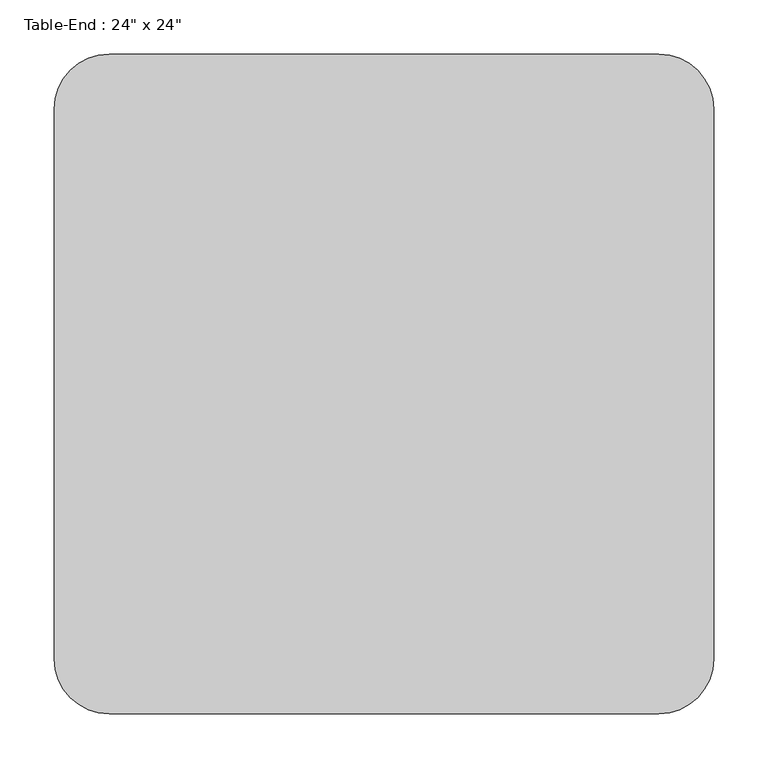
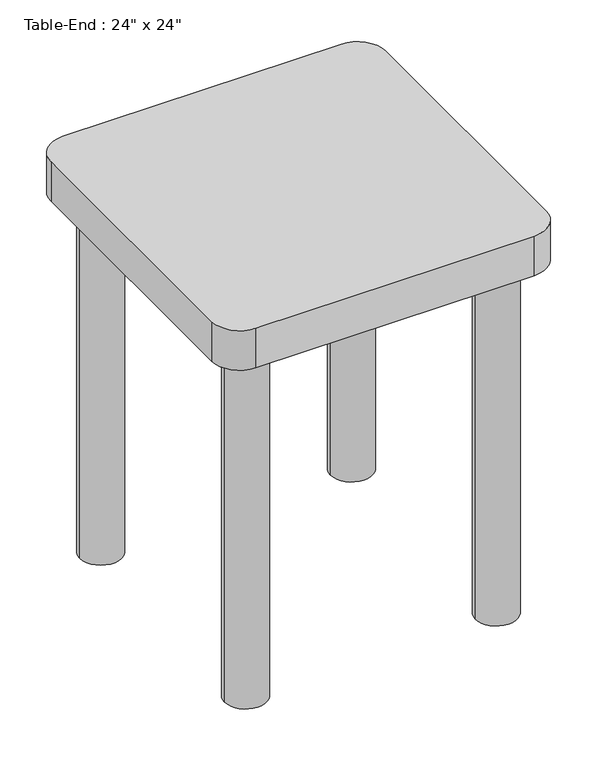
"""IFC4 building model written with IfcOpenShell, lengths in millimetres: furniture geometry."""

import ifcopenshell
import ifcopenshell.guid

model = None  # the IFC model being written
_history = None  # IfcOwnerHistory: only IFC2X3 demands one
_inside = {}  # id of a spatial element -> (the spatial element, [elements in it])
_under = {}  # id of a project, library or spatial element -> (it, [spatial elements below it])
_declared = {}  # id of a project -> (the project, [libraries it declares])
_typed = {}  # id of a type object -> (the type object, [elements of that type])
_made_of = {}  # id of a material, layer set ... -> (it, [elements and type objects made of it])


def new_model(schema):
    """Start an empty IFC model of exactly this schema.

    Asked for "IFC4X3", IfcOpenShell would pick the latest addendum, in which some entities
    have other attributes; the version numbers below select the first issue.
    IFC2X3 requires an IfcOwnerHistory on every rooted entity: one is made here for all.
    """
    global model, _history
    if schema == "IFC4X3":
        model = ifcopenshell.file(schema_version=(4, 3, 0, 0))
    else:
        model = ifcopenshell.file(schema=schema)
    _inside.clear()
    _under.clear()
    _declared.clear()
    _typed.clear()
    _made_of.clear()
    _history = None
    if model.schema == "IFC2X3":
        org = make("IfcOrganization", Name="unknown")
        user = make(
            "IfcPersonAndOrganization",
            ThePerson=make("IfcPerson", FamilyName="unknown"),
            TheOrganization=org,
        )
        app = make(
            "IfcApplication",
            ApplicationDeveloper=org,
            Version="unknown",
            ApplicationFullName="unknown",
            ApplicationIdentifier="unknown",
        )
        _history = make(
            "IfcOwnerHistory",
            OwningUser=user,
            OwningApplication=app,
            ChangeAction="ADDED",
            CreationDate=0,
        )
    return model


def make(cls, **values):
    """One entity of the class cls with the attributes given. An attribute that is None is left unset."""
    return model.create_entity(
        cls, **{name: value for name, value in values.items() if value is not None}
    )


def rooted(cls, **values):
    """An entity with a GlobalId (a new one), such as an element, a storey or a relation."""
    return make(cls, GlobalId=ifcopenshell.guid.new(), OwnerHistory=_history, **values)


def si_unit(unit_type, name, prefix=None):
    """IfcSIUnit, for example si_unit("LENGTHUNIT", "METRE", prefix="MILLI")."""
    return make("IfcSIUnit", UnitType=unit_type, Prefix=prefix, Name=name)


def assignment(units):
    """IfcUnitAssignment: the units of a project."""
    return None if units is None else make("IfcUnitAssignment", Units=units)


def point(xyz):
    """IfcCartesianPoint."""
    return None if xyz is None else make("IfcCartesianPoint", Coordinates=xyz)


def direction(xyz):
    """IfcDirection."""
    return None if xyz is None else make("IfcDirection", DirectionRatios=xyz)


def frame(location, z_axis=None, x_axis=None):
    """IfcAxis2Placement3D, a coordinate frame: its origin and axes. An axis left out is left unset."""
    return make(
        "IfcAxis2Placement3D",
        Location=point(location),
        Axis=direction(z_axis),
        RefDirection=direction(x_axis),
    )


def frame_2d(location, x_axis=None):
    """IfcAxis2Placement2D, a coordinate frame in the plane: its origin and x axis."""
    return make(
        "IfcAxis2Placement2D", Location=point(location), RefDirection=direction(x_axis)
    )


def origin():
    """The frame at (0, 0, 0) with its axes left unset."""
    return frame((0.0, 0.0, 0.0))


def origin_with_axes():
    """The frame at (0, 0, 0) with the z axis (0, 0, 1) and the x axis (1, 0, 0) written out."""
    return frame((0.0, 0.0, 0.0), z_axis=(0.0, 0.0, 1.0), x_axis=(1.0, 0.0, 0.0))


def place(relative_to, where):
    """IfcLocalPlacement: puts the frame where relative to a parent placement (None: the world)."""
    return make(
        "IfcLocalPlacement", PlacementRelTo=relative_to, RelativePlacement=where
    )


def context(
    kind, dimensions, precision=None, world=None, true_north=None, identifier=None
):
    """IfcGeometricRepresentationContext, for example the 3D "Model" context."""
    return make(
        "IfcGeometricRepresentationContext",
        ContextIdentifier=identifier,
        ContextType=kind,
        CoordinateSpaceDimension=dimensions,
        Precision=precision,
        WorldCoordinateSystem=world,
        TrueNorth=true_north,
    )


def project(units=None, contexts=None):
    """IfcProject with its units and contexts."""
    return rooted(
        "IfcProject",
        Name="project",
        RepresentationContexts=contexts,
        UnitsInContext=assignment(units),
    )


def spatial(cls, under=None, at=None, **own):
    """A site, building, storey or space (cls), placed at a placement, below another one or the project."""
    s = rooted(cls, ObjectPlacement=at, **own)
    if under is not None:
        _under.setdefault(under.id(), (under, []))[1].append(s)
    return s


def polyline(points):
    """IfcPolyline through the points."""
    return make("IfcPolyline", Points=[point(p) for p in points])


def circle_curve(where, radius):
    """IfcCircle in the frame where."""
    return make("IfcCircle", Position=where, Radius=radius)


def trimmed(basis, trim1, trim2, sense, master):
    """IfcTrimmedCurve: the piece of a basis curve between two trims."""
    return make(
        "IfcTrimmedCurve",
        BasisCurve=basis,
        Trim1=trim1,
        Trim2=trim2,
        SenseAgreement=sense,
        MasterRepresentation=master,
    )


def segment(curve, same_sense, transition):
    """IfcCompositeCurveSegment."""
    return make(
        "IfcCompositeCurveSegment",
        Transition=transition,
        SameSense=same_sense,
        ParentCurve=curve,
    )


def composite_curve(segments, self_intersect=None):
    """IfcCompositeCurve: segments joined end to end."""
    return make("IfcCompositeCurve", Segments=segments, SelfIntersect=self_intersect)


def outline(outer, holes=None, kind="AREA"):
    """IfcArbitraryClosedProfileDef: a profile drawn as a closed curve; with holes, ...WithVoids."""
    if holes is None:
        return make("IfcArbitraryClosedProfileDef", ProfileType=kind, OuterCurve=outer)
    return make(
        "IfcArbitraryProfileDefWithVoids",
        ProfileType=kind,
        OuterCurve=outer,
        InnerCurves=holes,
    )


def extrude(swept, where, along, depth):
    """IfcExtrudedAreaSolid: the profile swept, set in the frame where, extruded along a direction by depth."""
    return make(
        "IfcExtrudedAreaSolid",
        SweptArea=swept,
        Position=where,
        ExtrudedDirection=direction(along),
        Depth=depth,
    )


def shape(context_of_items, identifier, shape_type, items):
    """IfcShapeRepresentation: the items that make up one representation, for example the "Body"."""
    return make(
        "IfcShapeRepresentation",
        ContextOfItems=context_of_items,
        RepresentationIdentifier=identifier,
        RepresentationType=shape_type,
        Items=items,
    )


def source(mapping_origin, context_of_items, identifier, shape_type, items):
    """IfcRepresentationMap: a shape defined once, which mapped items show again and again."""
    return make(
        "IfcRepresentationMap",
        MappingOrigin=mapping_origin,
        MappedRepresentation=shape(context_of_items, identifier, shape_type, items),
    )


def transform(
    local_origin,
    x_axis=None,
    y_axis=None,
    z_axis=None,
    scale=None,
    scale2=None,
    scale3=None,
    uniform=True,
):
    """IfcCartesianTransformationOperator3D, or its non-uniform kind. x_axis, y_axis, z_axis: its Axis1, 2, 3."""
    if uniform:
        return make(
            "IfcCartesianTransformationOperator3D",
            Axis1=direction(x_axis),
            Axis2=direction(y_axis),
            LocalOrigin=point(local_origin),
            Scale=scale,
            Axis3=direction(z_axis),
        )
    return make(
        "IfcCartesianTransformationOperator3DnonUniform",
        Axis1=direction(x_axis),
        Axis2=direction(y_axis),
        LocalOrigin=point(local_origin),
        Scale=scale,
        Axis3=direction(z_axis),
        Scale2=scale2,
        Scale3=scale3,
    )


def mapped(mapping_source, mapping_target):
    """IfcMappedItem: shows the shape of a source again, moved by a transform."""
    return make(
        "IfcMappedItem", MappingSource=mapping_source, MappingTarget=mapping_target
    )


def made_of(thing, what):
    """Note that an element or type object is made of a material, layer set ...; save() writes the relation."""
    if what is not None:
        _made_of.setdefault(what.id(), (what, []))[1].append(thing)
    return thing


def element(
    cls,
    number,
    at=None,
    inside=None,
    cuts=None,
    type_object=None,
    material=None,
    context=None,
    identifier="Body",
    shape_type=None,
    held_by="IfcProductDefinitionShape",
    body=None,
    shapes=None,
    **own,
):
    """One element of the class cls, such as IfcWall. Its Tag is "e" and its number.

    at: its placement. inside: the storey or other place that contains it. cuts: it is an
    opening in that element (IfcRelVoidsElement). A single representation is given by context,
    identifier, shape_type and body (its items); several are given by shapes. held_by: the class
    of the entity that holds the representations. save() writes the other relations.
    """
    e = rooted(cls, Tag="e%d" % number, ObjectPlacement=at, **own)
    if body is not None:
        shapes = [shape(context, identifier, shape_type, body)]
    if shapes is not None:
        e.Representation = make(held_by, Representations=shapes)
    if inside is not None:
        _inside.setdefault(inside.id(), (inside, []))[1].append(e)
    if cuts is not None:
        rooted(
            "IfcRelVoidsElement", RelatingBuildingElement=cuts, RelatedOpeningElement=e
        )
    if type_object is not None:
        _typed.setdefault(type_object.id(), (type_object, []))[1].append(e)
    return made_of(e, material)


def aggregate(whole, parts):
    """IfcRelAggregates: a whole, such as a stair, and the parts it consists of."""
    return rooted("IfcRelAggregates", RelatingObject=whole, RelatedObjects=parts)


def save(model, path):
    """Write the relations noted so far, then the file.

    IfcRelAggregates (storeys below a building ...), IfcRelContainedInSpatialStructure (elements
    in a storey), IfcRelDefinesByType, IfcRelAssociatesMaterial and IfcRelDeclares: one each for
    every whole, place, type object, material and project.
    """
    for whole, parts in _under.values():
        aggregate(whole, parts)
    for where, things in _inside.values():
        rooted(
            "IfcRelContainedInSpatialStructure",
            RelatedElements=things,
            RelatingStructure=where,
        )
    for kind, things in _typed.values():
        rooted("IfcRelDefinesByType", RelatedObjects=things, RelatingType=kind)
    for what, things in _made_of.values():
        rooted("IfcRelAssociatesMaterial", RelatedObjects=things, RelatingMaterial=what)
    for by, libraries in _declared.values():
        rooted("IfcRelDeclares", RelatingContext=by, RelatedDefinitions=libraries)
    model.write(path)


def furniture_bcf351fa(model_context):
    return source(origin(), model_context, "Body", "SweptSolid", [
        extrude(outline(composite_curve([segment(polyline([(562.5336303, -152.4), (54.5336303, -152.4)]), True, "CONTINUOUS"), segment(trimmed(circle_curve(frame_2d((54.5336303, -101.6)), 50.8), [point((54.5336303, -152.4))], [point((3.7336303, -101.6))], False, "CARTESIAN"), True, "CONTINUOUS"), segment(polyline([(3.7336303, -101.6), (3.7336303, 406.4)]), True, "CONTINUOUS"), segment(trimmed(circle_curve(frame_2d((54.5336303, 406.4)), 50.8), [point((3.7336303, 406.4))], [point((54.5336303, 457.2))], False, "CARTESIAN"), True, "CONTINUOUS"), segment(polyline([(54.5336303, 457.2), (562.5336303, 457.2)]), True, "CONTINUOUS"), segment(trimmed(circle_curve(frame_2d((562.5336303, 406.4)), 50.8), [point((562.5336303, 457.2))], [point((613.3336303, 406.4))], False, "CARTESIAN"), True, "CONTINUOUS"), segment(polyline([(613.3336303, 406.4), (613.3336303, -101.6)]), True, "CONTINUOUS"), segment(trimmed(circle_curve(frame_2d((562.5336303, -101.6)), 50.8), [point((613.3336303, -101.6))], [point((562.5336303, -152.4))], False, "CARTESIAN"), True, "CONTINUOUS")], self_intersect=False)), frame((0.0, 0.0, 685.8), z_axis=(0.0, 0.0, 1.0), x_axis=(1.0, 0.0, 0.0)), (0.0, 0.0, 1.0), 76.2),
        extrude(outline(composite_curve([segment(trimmed(circle_curve(frame_2d((79.9336303, 381.0)), 38.1), [point((41.8336303, 381.0))], [point((118.0336303, 381.0))], False, "CARTESIAN"), True, "CONTINUOUS"), segment(trimmed(circle_curve(frame_2d((79.9336303, 381.0)), 38.1), [point((118.0336303, 381.0))], [point((41.8336303, 381.0))], False, "CARTESIAN"), True, "CONTINUOUS")], self_intersect=False)), origin_with_axes(), (0.0, 0.0, 1.0), 685.8),
        extrude(outline(composite_curve([segment(trimmed(circle_curve(frame_2d((79.9336303, -76.2)), 38.1), [point((41.8336303, -76.2))], [point((118.0336303, -76.2))], False, "CARTESIAN"), True, "CONTINUOUS"), segment(trimmed(circle_curve(frame_2d((79.9336303, -76.2)), 38.1), [point((118.0336303, -76.2))], [point((41.8336303, -76.2))], False, "CARTESIAN"), True, "CONTINUOUS")], self_intersect=False)), origin_with_axes(), (0.0, 0.0, 1.0), 685.8),
        extrude(outline(composite_curve([segment(trimmed(circle_curve(frame_2d((537.1336303, -76.2)), 38.1), [point((499.0336303, -76.2))], [point((575.2336303, -76.2))], False, "CARTESIAN"), True, "CONTINUOUS"), segment(trimmed(circle_curve(frame_2d((537.1336303, -76.2)), 38.1), [point((575.2336303, -76.2))], [point((499.0336303, -76.2))], False, "CARTESIAN"), True, "CONTINUOUS")], self_intersect=False)), origin_with_axes(), (0.0, 0.0, 1.0), 685.8),
        extrude(outline(composite_curve([segment(trimmed(circle_curve(frame_2d((537.1336303, 381.0)), 38.1), [point((499.0336303, 381.0))], [point((575.2336303, 381.0))], False, "CARTESIAN"), True, "CONTINUOUS"), segment(trimmed(circle_curve(frame_2d((537.1336303, 381.0)), 38.1), [point((575.2336303, 381.0))], [point((499.0336303, 381.0))], False, "CARTESIAN"), True, "CONTINUOUS")], self_intersect=False)), origin_with_axes(), (0.0, 0.0, 1.0), 685.8),
    ])


if __name__ == "__main__":
    model = new_model("IFC4")
    model_context = context("Model", 3, world=origin())
    ifc_project = project(units=[si_unit("LENGTHUNIT", "METRE", prefix="MILLI")], contexts=[model_context])
    site = spatial("IfcSite", under=ifc_project)
    building = spatial("IfcBuilding", under=site)
    placement = place(None, origin())
    furniture_shape = furniture_bcf351fa(model_context)
    element("IfcFurniture", 1, ObjectType="Table-End : 24\" x 24\"", at=placement, inside=building, context=model_context, shape_type="MappedRepresentation", body=[
        mapped(furniture_shape, transform((0.0, 0.0, 0.0), x_axis=(1.0, 0.0, 0.0), y_axis=(0.0, 1.0, 0.0), z_axis=(0.0, 0.0, 1.0))),
    ])
    save(model, "model.ifc")

# Revit data of these elements
# Type "Table-End : 24\" x 24\""
#   Model = "End Table"
#   Manufacturer = "Acme Funriture"
#   Assembly Code = "E2020200"
#   Height = 2' - 6"
#   Length = 2' - 0"
#   Width = 2' - 0"
#   Base Material = Birch
#   Top Material = Laminate, Blue, Matte
#   Default Elevation = 0
# Element 1 (IfcFurniture, "Table-End : 24\" x 24\"")
#   Materials on its faces: "Laminate, Blue, Matte", "Birch"
# Materials
#   "Birch": class "Wood", colour RGB 172 132 95, transparency 0, Description = "Betula Alleghaniensis", Cost = 0
#   "Laminate, Blue, Matte": class "Plastic", colour RGB 85 101 155, transparency 0, Description = "Plastic Laminate - Blue, Matte", Cost = 0
